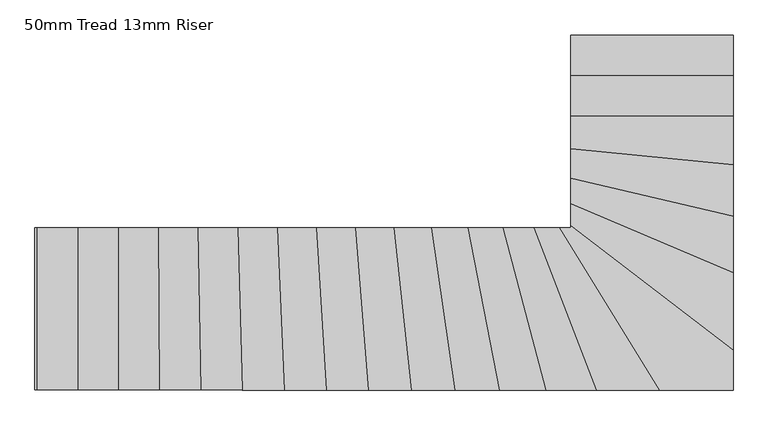
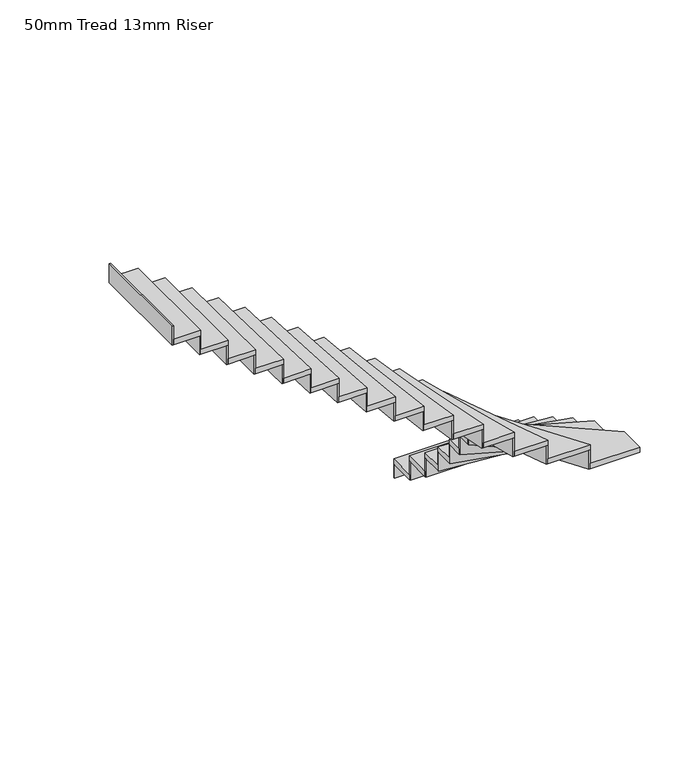
"""IFC4 building model written with IfcOpenShell, lengths in millimetres: stair flight geometry, 50mm Tread 13mm Riser."""

from ifc_helpers import new_model, si_unit, frame, origin, origin_with_axes, place, context, project, spatial, polyline, outline, extrude, source, transform, mapped, element, save


def stair_flight_50mm_tread_13mm_riser_dd38c772(model_context):
    return source(origin(), model_context, "Body", "SweptSolid", [
        extrude(outline(polyline([(22436.9270386, -2702.5996592), (22436.9270386, -2690.0996592), (23436.9270386, -2690.0996592), (23436.9270386, -2702.5996592), (22436.9270386, -2702.5996592)])), origin_with_axes(), (0.0, 0.0, 1.0), 131.8181818),
        extrude(outline(polyline([(23436.9270386, -2940.0996592), (22436.9270386, -2940.0996592), (22436.9270386, -2690.0996592), (23436.9270386, -2690.0996592), (23436.9270386, -2940.0996592)])), frame((0.0, 0.0, 131.8181818), z_axis=(0.0, 0.0, 1.0), x_axis=(1.0, 0.0, 0.0)), (0.0, 0.0, 1.0), 50.0),
        extrude(outline(polyline([(22436.9270386, -2952.5996592), (22436.9270386, -2940.0996592), (23436.9270386, -2940.0996592), (23436.9270386, -2952.5996592), (22436.9270386, -2952.5996592)])), frame((0.0, 0.0, 131.8181818), z_axis=(0.0, 0.0, 1.0), x_axis=(1.0, 0.0, 0.0)), (0.0, 0.0, 1.0), 181.8181818),
        extrude(outline(polyline([(23436.9270386, -3190.0996592), (22436.9270386, -3190.0996592), (22436.9270386, -2940.0996592), (23436.9270386, -2940.0996592), (23436.9270386, -3190.0996592)])), frame((0.0, 0.0, 313.6363636), z_axis=(0.0, 0.0, 1.0), x_axis=(1.0, 0.0, 0.0)), (0.0, 0.0, 1.0), 50.0),
        extrude(outline(polyline([(22436.9270386, -3202.5996592), (22436.9270386, -3190.0996592), (23436.9270386, -3190.0996592), (23436.9270386, -3202.5996592), (22436.9270386, -3202.5996592)])), frame((0.0, 0.0, 313.6363636), z_axis=(0.0, 0.0, 1.0), x_axis=(1.0, 0.0, 0.0)), (0.0, 0.0, 1.0), 181.8181818),
        extrude(outline(polyline([(23436.9270386, -3489.5124544), (22436.9270386, -3390.686864), (22436.9270386, -3190.0996592), (23436.9270386, -3190.0996592), (23436.9270386, -3489.5124544)])), frame((0.0, 0.0, 495.4545455), z_axis=(0.0, 0.0, 1.0), x_axis=(1.0, 0.0, 0.0)), (0.0, 0.0, 1.0), 50.0),
        extrude(outline(polyline([(22436.9270386, -3403.2477563), (22436.9270386, -3390.686864), (23436.9270386, -3489.5124544), (23436.9270386, -3502.0733467), (22436.9270386, -3403.2477563)])), frame((0.0, 0.0, 495.4545455), z_axis=(0.0, 0.0, 1.0), x_axis=(1.0, 0.0, 0.0)), (0.0, 0.0, 1.0), 181.8181818),
        extrude(outline(polyline([(23436.9270386, -3806.6031161), (22436.9270386, -3573.5962022), (22436.9270386, -3390.686864), (23436.9270386, -3489.5124544), (23436.9270386, -3806.6031161)])), frame((0.0, 0.0, 677.2727273), z_axis=(0.0, 0.0, 1.0), x_axis=(1.0, 0.0, 0.0)), (0.0, 0.0, 1.0), 50.0),
        extrude(outline(polyline([(22436.9270386, -3586.4310438), (22436.9270386, -3573.5962022), (23436.9270386, -3806.6031161), (23436.9270386, -3819.4379578), (22436.9270386, -3586.4310438)])), frame((0.0, 0.0, 677.2727273), z_axis=(0.0, 0.0, 1.0), x_axis=(1.0, 0.0, 0.0)), (0.0, 0.0, 1.0), 181.8181818),
        extrude(outline(polyline([(23436.9270386, -4155.1194815), (22436.9270386, -3728.4987988), (22436.9270386, -3573.5962022), (23436.9270386, -3806.6031161), (23436.9270386, -4155.1194815)])), frame((0.0, 0.0, 859.0909091), z_axis=(0.0, 0.0, 1.0), x_axis=(1.0, 0.0, 0.0)), (0.0, 0.0, 1.0), 50.0),
        extrude(outline(polyline([(22436.9270386, -3742.0888066), (22436.9270386, -3728.4987988), (23436.9270386, -4155.1194815), (23436.9270386, -4168.7094894), (22436.9270386, -3742.0888066)])), frame((0.0, 0.0, 859.0909091), z_axis=(0.0, 0.0, 1.0), x_axis=(1.0, 0.0, 0.0)), (0.0, 0.0, 1.0), 181.8181818),
        extrude(outline(polyline([(23436.9270386, -4629.7583436), (22436.9270386, -3863.2317902), (22436.9270386, -3728.4987988), (23436.9270386, -4155.1194815), (23436.9270386, -4629.7583436)])), frame((0.0, 0.0, 1040.9090909), z_axis=(0.0, 0.0, 1.0), x_axis=(1.0, 0.0, 0.0)), (0.0, 0.0, 1.0), 50.0),
        extrude(outline(polyline([(22436.9270386, -3878.9816065), (22436.9270386, -3863.2317902), (23436.9270386, -4629.7583436), (23436.9270386, -4645.5081599), (22436.9270386, -3878.9816065)])), frame((0.0, 0.0, 1040.9090909), z_axis=(0.0, 0.0, 1.0), x_axis=(1.0, 0.0, 0.0)), (0.0, 0.0, 1.0), 181.8181818),
        extrude(outline(polyline([(22983.3050877, -4876.2808257), (22366.119393, -3876.2808257), (22436.9270386, -3876.2808257), (22436.9270386, -3863.2317902), (23436.9270386, -4629.7583436), (23436.9270386, -4876.2808257), (22983.3050877, -4876.2808257)])), frame((0.0, 0.0, 1222.7272727), z_axis=(0.0, 0.0, 1.0), x_axis=(1.0, 0.0, 0.0)), (0.0, 0.0, 1.0), 50.0),
        extrude(outline(polyline([(22351.4303336, -3876.2808257), (22366.119393, -3876.2808257), (22983.3050877, -4876.2808257), (22968.6160283, -4876.2808257), (22351.4303336, -3876.2808257)])), frame((0.0, 0.0, 1222.7272727), z_axis=(0.0, 0.0, 1.0), x_axis=(1.0, 0.0, 0.0)), (0.0, 0.0, 1.0), 181.8181818),
        extrude(outline(polyline([(22592.8894543, -4876.2808257), (22208.3187485, -3876.2808257), (22366.119393, -3876.2808257), (22983.3050877, -4876.2808257), (22592.8894543, -4876.2808257)])), frame((0.0, 0.0, 1404.5454545), z_axis=(0.0, 0.0, 1.0), x_axis=(1.0, 0.0, 0.0)), (0.0, 0.0, 1.0), 50.0),
        extrude(outline(polyline([(22194.9262679, -3876.2808257), (22208.3187485, -3876.2808257), (22592.8894543, -4876.2808257), (22579.4969737, -4876.2808257), (22194.9262679, -3876.2808257)])), frame((0.0, 0.0, 1404.5454545), z_axis=(0.0, 0.0, 1.0), x_axis=(1.0, 0.0, 0.0)), (0.0, 0.0, 1.0), 181.8181818),
        extrude(outline(polyline([(22283.5569946, -4876.2808257), (22017.6512081, -3876.2808257), (22208.3187485, -3876.2808257), (22592.8894543, -4876.2808257), (22283.5569946, -4876.2808257)])), frame((0.0, 0.0, 1586.3636364), z_axis=(0.0, 0.0, 1.0), x_axis=(1.0, 0.0, 0.0)), (0.0, 0.0, 1.0), 50.0),
        extrude(outline(polyline([(22004.7168433, -3876.2808257), (22017.6512081, -3876.2808257), (22283.5569946, -4876.2808257), (22270.6226297, -4876.2808257), (22004.7168433, -3876.2808257)])), frame((0.0, 0.0, 1586.3636364), z_axis=(0.0, 0.0, 1.0), x_axis=(1.0, 0.0, 0.0)), (0.0, 0.0, 1.0), 181.8181818),
        extrude(outline(polyline([(21997.1472408, -4876.2808257), (21804.0609619, -3876.2808257), (22017.6512081, -3876.2808257), (22283.5569946, -4876.2808257), (21997.1472408, -4876.2808257)])), frame((0.0, 0.0, 1768.1818182), z_axis=(0.0, 0.0, 1.0), x_axis=(1.0, 0.0, 0.0)), (0.0, 0.0, 1.0), 50.0),
        extrude(outline(polyline([(21791.3300797, -3876.2808257), (21804.0609619, -3876.2808257), (21997.1472408, -4876.2808257), (21984.4163587, -4876.2808257), (21791.3300797, -3876.2808257)])), frame((0.0, 0.0, 1768.1818182), z_axis=(0.0, 0.0, 1.0), x_axis=(1.0, 0.0, 0.0)), (0.0, 0.0, 1.0), 181.8181818),
        extrude(outline(polyline([(21722.5267953, -4876.2808257), (21578.6814075, -3876.2808257), (21804.0609619, -3876.2808257), (21997.1472408, -4876.2808257), (21722.5267953, -4876.2808257)])), frame((0.0, 0.0, 1950.0), z_axis=(0.0, 0.0, 1.0), x_axis=(1.0, 0.0, 0.0)), (0.0, 0.0, 1.0), 50.0),
        extrude(outline(polyline([(21566.0527478, -3876.2808257), (21578.6814075, -3876.2808257), (21722.5267953, -4876.2808257), (21709.8981356, -4876.2808257), (21566.0527478, -3876.2808257)])), frame((0.0, 0.0, 1950.0), z_axis=(0.0, 0.0, 1.0), x_axis=(1.0, 0.0, 0.0)), (0.0, 0.0, 1.0), 181.8181818),
        extrude(outline(polyline([(21454.7675265, -4876.2808257), (21346.4406763, -3876.2808257), (21578.6814075, -3876.2808257), (21722.5267953, -4876.2808257), (21454.7675265, -4876.2808257)])), frame((0.0, 0.0, 2131.8181818), z_axis=(0.0, 0.0, 1.0), x_axis=(1.0, 0.0, 0.0)), (0.0, 0.0, 1.0), 50.0),
        extrude(outline(polyline([(21333.8675483, -3876.2808257), (21346.4406763, -3876.2808257), (21454.7675265, -4876.2808257), (21442.1943985, -4876.2808257), (21333.8675483, -3876.2808257)])), frame((0.0, 0.0, 2131.8181818), z_axis=(0.0, 0.0, 1.0), x_axis=(1.0, 0.0, 0.0)), (0.0, 0.0, 1.0), 181.8181818),
        extrude(outline(polyline([(21191.3521077, -4876.2808257), (21109.8560951, -3876.2808257), (21346.4406763, -3876.2808257), (21454.7675265, -4876.2808257), (21191.3521077, -4876.2808257)])), frame((0.0, 0.0, 2313.6363636), z_axis=(0.0, 0.0, 1.0), x_axis=(1.0, 0.0, 0.0)), (0.0, 0.0, 1.0), 50.0),
        extrude(outline(polyline([(21097.3146538, -3876.2808257), (21109.8560951, -3876.2808257), (21191.3521077, -4876.2808257), (21178.8106664, -4876.2808257), (21097.3146538, -3876.2808257)])), frame((0.0, 0.0, 2313.6363636), z_axis=(0.0, 0.0, 1.0), x_axis=(1.0, 0.0, 0.0)), (0.0, 0.0, 1.0), 181.8181818),
        extrude(outline(polyline([(20930.8604759, -4876.2808257), (20870.3477268, -3876.2808257), (21109.8560951, -3876.2808257), (21191.3521077, -4876.2808257), (20930.8604759, -4876.2808257)])), frame((0.0, 0.0, 2495.4545455), z_axis=(0.0, 0.0, 1.0), x_axis=(1.0, 0.0, 0.0)), (0.0, 0.0, 1.0), 50.0),
        extrude(outline(polyline([(20857.8248615, -3876.2808257), (20870.3477268, -3876.2808257), (20930.8604759, -4876.2808257), (20918.3376106, -4876.2808257), (20857.8248615, -3876.2808257)])), frame((0.0, 0.0, 2495.4545455), z_axis=(0.0, 0.0, 1.0), x_axis=(1.0, 0.0, 0.0)), (0.0, 0.0, 1.0), 181.8181818),
        extrude(outline(polyline([(20672.4307285, -4876.2808257), (20628.7774743, -3876.2808257), (20870.3477268, -3876.2808257), (20930.8604759, -4876.2808257), (20672.4307285, -4876.2808257)])), frame((0.0, 0.0, 2677.2727273), z_axis=(0.0, 0.0, 1.0), x_axis=(1.0, 0.0, 0.0)), (0.0, 0.0, 1.0), 50.0),
        extrude(outline(polyline([(20616.2655699, -3876.2808257), (20628.7774743, -3876.2808257), (20672.4307285, -4876.2808257), (20659.9188241, -4876.2808257), (20616.2655699, -3876.2808257)])), frame((0.0, 0.0, 2677.2727273), z_axis=(0.0, 0.0, 1.0), x_axis=(1.0, 0.0, 0.0)), (0.0, 0.0, 1.0), 181.8181818),
        extrude(outline(polyline([(20415.5094256, -4876.2808257), (20385.6987771, -3876.2808257), (20628.7774743, -3876.2808257), (20672.4307285, -4876.2808257), (20415.5094256, -4876.2808257)])), frame((0.0, 0.0, 2859.0909091), z_axis=(0.0, 0.0, 1.0), x_axis=(1.0, 0.0, 0.0)), (0.0, 0.0, 1.0), 50.0),
        extrude(outline(polyline([(20373.1932241, -3876.2808257), (20385.6987771, -3876.2808257), (20415.5094256, -4876.2808257), (20403.0038727, -4876.2808257), (20373.1932241, -3876.2808257)])), frame((0.0, 0.0, 2859.0909091), z_axis=(0.0, 0.0, 1.0), x_axis=(1.0, 0.0, 0.0)), (0.0, 0.0, 1.0), 181.8181818),
        extrude(outline(polyline([(20159.7249299, -4876.2808257), (20141.4832729, -3876.2808257), (20385.6987771, -3876.2808257), (20415.5094256, -4876.2808257), (20159.7249299, -4876.2808257)])), frame((0.0, 0.0, 3040.9090909), z_axis=(0.0, 0.0, 1.0), x_axis=(1.0, 0.0, 0.0)), (0.0, 0.0, 1.0), 50.0),
        extrude(outline(polyline([(20128.9811933, -3876.2808257), (20141.4832729, -3876.2808257), (20159.7249299, -4876.2808257), (20147.2228503, -4876.2808257), (20128.9811933, -3876.2808257)])), frame((0.0, 0.0, 3040.9090909), z_axis=(0.0, 0.0, 1.0), x_axis=(1.0, 0.0, 0.0)), (0.0, 0.0, 1.0), 181.8181818),
        extrude(outline(polyline([(19904.8184199, -4876.2808257), (19896.3897829, -3876.2808257), (20141.4832729, -3876.2808257), (20159.7249299, -4876.2808257), (19904.8184199, -4876.2808257)])), frame((0.0, 0.0, 3222.7272727), z_axis=(0.0, 0.0, 1.0), x_axis=(1.0, 0.0, 0.0)), (0.0, 0.0, 1.0), 50.0),
        extrude(outline(polyline([(19883.8893389, -3876.2808257), (19896.3897829, -3876.2808257), (19904.8184199, -4876.2808257), (19892.3179759, -4876.2808257), (19883.8893389, -3876.2808257)])), frame((0.0, 0.0, 3222.7272727), z_axis=(0.0, 0.0, 1.0), x_axis=(1.0, 0.0, 0.0)), (0.0, 0.0, 1.0), 181.8181818),
        extrude(outline(polyline([(19650.6041014, -4876.2808257), (19650.6041014, -3876.2808257), (19896.3897829, -3876.2808257), (19904.8184199, -4876.2808257), (19650.6041014, -4876.2808257)])), frame((0.0, 0.0, 3404.5454545), z_axis=(0.0, 0.0, 1.0), x_axis=(1.0, 0.0, 0.0)), (0.0, 0.0, 1.0), 50.0),
        extrude(outline(polyline([(19638.1041014, -3876.2808257), (19650.6041014, -3876.2808257), (19650.6041014, -4876.2808257), (19638.1041014, -4876.2808257), (19638.1041014, -3876.2808257)])), frame((0.0, 0.0, 3404.5454545), z_axis=(0.0, 0.0, 1.0), x_axis=(1.0, 0.0, 0.0)), (0.0, 0.0, 1.0), 181.8181818),
        extrude(outline(polyline([(19400.6041014, -4876.2808257), (19400.6041014, -3876.2808257), (19650.6041014, -3876.2808257), (19650.6041014, -4876.2808257), (19400.6041014, -4876.2808257)])), frame((0.0, 0.0, 3586.3636364), z_axis=(0.0, 0.0, 1.0), x_axis=(1.0, 0.0, 0.0)), (0.0, 0.0, 1.0), 50.0),
        extrude(outline(polyline([(19388.1041014, -3876.2808257), (19400.6041014, -3876.2808257), (19400.6041014, -4876.2808257), (19388.1041014, -4876.2808257), (19388.1041014, -3876.2808257)])), frame((0.0, 0.0, 3586.3636364), z_axis=(0.0, 0.0, 1.0), x_axis=(1.0, 0.0, 0.0)), (0.0, 0.0, 1.0), 181.8181818),
        extrude(outline(polyline([(19138.1041014, -3876.2808257), (19150.6041014, -3876.2808257), (19150.6041014, -4876.2808257), (19138.1041014, -4876.2808257), (19138.1041014, -3876.2808257)])), frame((0.0, 0.0, 3768.1818182), z_axis=(0.0, 0.0, 1.0), x_axis=(1.0, 0.0, 0.0)), (0.0, 0.0, 1.0), 181.8181818),
        extrude(outline(polyline([(19150.6041014, -4876.2808257), (19150.6041014, -3876.2808257), (19400.6041014, -3876.2808257), (19400.6041014, -4876.2808257), (19150.6041014, -4876.2808257)])), frame((0.0, 0.0, 3768.1818182), z_axis=(0.0, 0.0, 1.0), x_axis=(1.0, 0.0, 0.0)), (0.0, 0.0, 1.0), 50.0),
    ])


if __name__ == "__main__":
    model = new_model("IFC4")
    model_context = context("Model", 3, world=origin())
    ifc_project = project(units=[si_unit("LENGTHUNIT", "METRE", prefix="MILLI")], contexts=[model_context])
    site = spatial("IfcSite", under=ifc_project)
    building = spatial("IfcBuilding", under=site)
    placement = place(None, origin())
    stair_flight_50mm_tread_13mm_riser_shape = stair_flight_50mm_tread_13mm_riser_dd38c772(model_context)
    element("IfcStairFlight", 1, ObjectType="50mm Tread 13mm Riser", at=placement, inside=building, context=model_context, shape_type="MappedRepresentation", body=[
        mapped(stair_flight_50mm_tread_13mm_riser_shape, transform((0.0, 0.0, 0.0), x_axis=(1.0, 0.0, 0.0), y_axis=(0.0, 1.0, 0.0), z_axis=(0.0, 0.0, 1.0))),
    ])
    save(model, "model.ifc")
